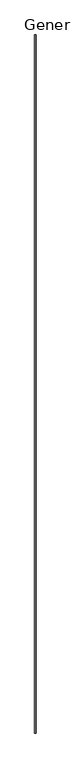
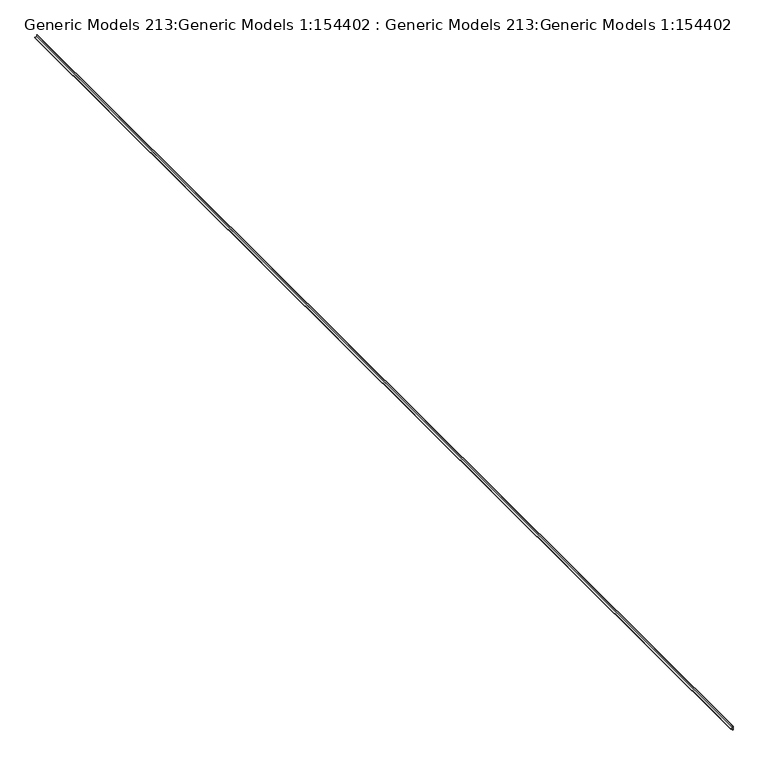
"""IFC4 building model written with IfcOpenShell, lengths in millimetres: proxy geometry, Generic Models 213:Generic Models 1:154402 : Generic Models 213:Generic Models 1:154402."""

from ifc_helpers import new_model, si_unit, frame, origin, place, context, project, spatial, polyline, outline, extrude, source, transform, mapped, element, save


def generic_models_213_generic_models_1_154402_generic_models_ceb327b4(model_context):
    return source(origin(), model_context, "Body", "SweptSolid", [
        extrude(outline(polyline([(3078.48, -6667.0793913), (3117.85, -6667.0793913), (3117.85, -6668.3493913), (3098.8, -6668.3493913), (3098.8, -6689.3043913), (3094.0502, -6689.3043913), (3094.0502, -6688.0343913), (3097.53, -6688.0343913), (3097.53, -6668.3493913), (3078.48, -6668.3493913), (3078.48, -6667.0793913)])), frame((0.0, -12719.9974793, 0.0), z_axis=(0.0, 1.0, 0.0), x_axis=(0.0, 0.0, 1.0)), (0.0, 0.0, 1.0), 12446.0),
    ])


if __name__ == "__main__":
    model = new_model("IFC4")
    model_context = context("Model", 3, world=origin())
    ifc_project = project(units=[si_unit("LENGTHUNIT", "METRE", prefix="MILLI")], contexts=[model_context])
    site = spatial("IfcSite", under=ifc_project)
    building = spatial("IfcBuilding", under=site)
    placement = place(None, origin())
    generic_models_213_generic_models_1_154402_generic_models_shape = generic_models_213_generic_models_1_154402_generic_models_ceb327b4(model_context)
    element("IfcBuildingElementProxy", 1, Name="Generic Models 213:Generic Models 1:154402 : Generic Models 213:Generic Models 1:154402", ObjectType="Generic Models 213:Generic Models 1:154402 : Generic Models 213:Generic Models 1:154402", at=placement, inside=building, context=model_context, shape_type="MappedRepresentation", body=[
        mapped(generic_models_213_generic_models_1_154402_generic_models_shape, transform((0.0, 0.0, 0.0), x_axis=(1.0, 0.0, 0.0), y_axis=(0.0, 1.0, 0.0), z_axis=(0.0, 0.0, 1.0))),
    ])
    save(model, "model.ifc")

# Revit data of these elements
# Type "Generic Models 213:Generic Models 1:154402 : Generic Models 213:Generic Models 1:154402"
#   NameOverride = "Generic Models 213:Generic Models 1:154402"
#   ObjectTypeOverride = "Generic Models 213:Generic Models 1"
#   Reference = "Generic Models 1"
#   Category = "Generic Models"
#   Tag = "154402"
# Element 1 (IfcBuildingElementProxy, "Generic Models 213:Generic Models 1:154402 : Generic Models 213:Generic Models 1:154402")
#   Materials on its faces: "_ 16 GA. COPPER VENTED T REVEAL BEAD (CONT. AROUND PERIMETER OF BEAM) 2987"
# Materials
#   "_ 16 GA. COPPER VENTED T REVEAL BEAD (CONT. AROUND PERIMETER OF BEAM) 2987": class "Unassigned", colour RGB 253 192 103, transparency 0
